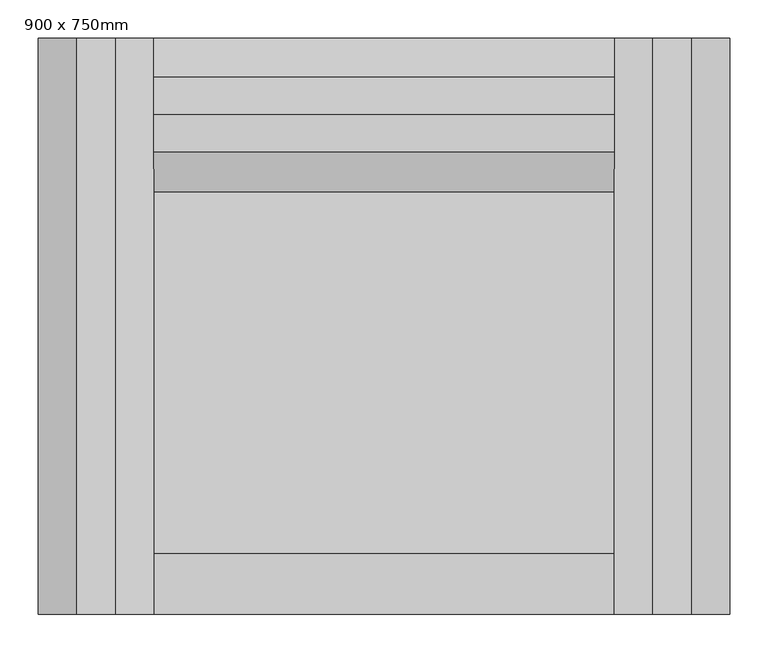
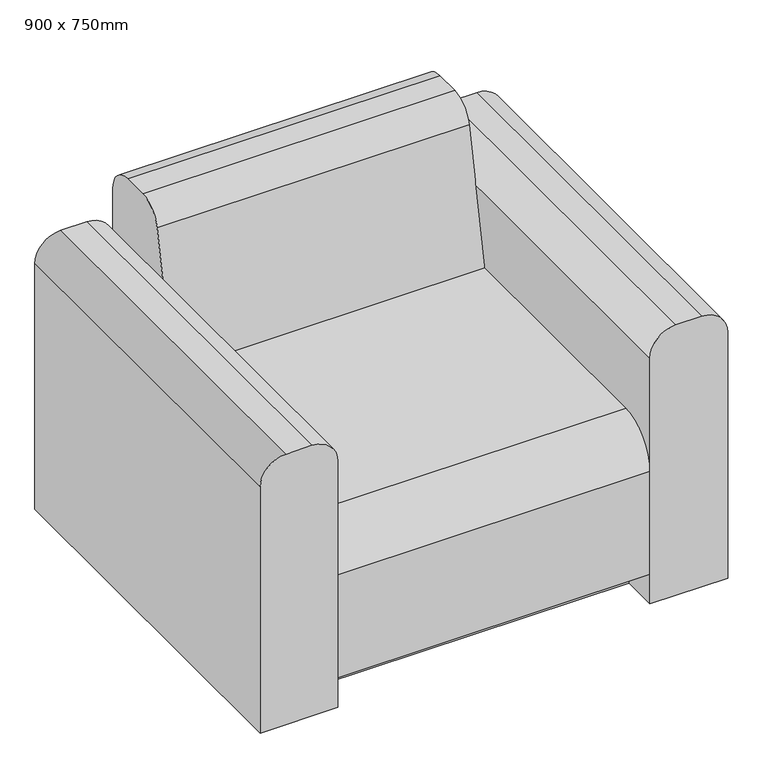
"""IFC4 building model written with IfcOpenShell, lengths in millimetres: furniture geometry, ソファ－I型 : 900 x 750mm."""

import ifcopenshell
import ifcopenshell.guid

model = None  # the IFC model being written
_history = None  # IfcOwnerHistory: only IFC2X3 demands one
_inside = {}  # id of a spatial element -> (the spatial element, [elements in it])
_under = {}  # id of a project, library or spatial element -> (it, [spatial elements below it])
_declared = {}  # id of a project -> (the project, [libraries it declares])
_typed = {}  # id of a type object -> (the type object, [elements of that type])
_made_of = {}  # id of a material, layer set ... -> (it, [elements and type objects made of it])


def new_model(schema):
    """Start an empty IFC model of exactly this schema.

    Asked for "IFC4X3", IfcOpenShell would pick the latest addendum, in which some entities
    have other attributes; the version numbers below select the first issue.
    IFC2X3 requires an IfcOwnerHistory on every rooted entity: one is made here for all.
    """
    global model, _history
    if schema == "IFC4X3":
        model = ifcopenshell.file(schema_version=(4, 3, 0, 0))
    else:
        model = ifcopenshell.file(schema=schema)
    _inside.clear()
    _under.clear()
    _declared.clear()
    _typed.clear()
    _made_of.clear()
    _history = None
    if model.schema == "IFC2X3":
        org = make("IfcOrganization", Name="unknown")
        user = make(
            "IfcPersonAndOrganization",
            ThePerson=make("IfcPerson", FamilyName="unknown"),
            TheOrganization=org,
        )
        app = make(
            "IfcApplication",
            ApplicationDeveloper=org,
            Version="unknown",
            ApplicationFullName="unknown",
            ApplicationIdentifier="unknown",
        )
        _history = make(
            "IfcOwnerHistory",
            OwningUser=user,
            OwningApplication=app,
            ChangeAction="ADDED",
            CreationDate=0,
        )
    return model


def make(cls, **values):
    """One entity of the class cls with the attributes given. An attribute that is None is left unset."""
    return model.create_entity(
        cls, **{name: value for name, value in values.items() if value is not None}
    )


def rooted(cls, **values):
    """An entity with a GlobalId (a new one), such as an element, a storey or a relation."""
    return make(cls, GlobalId=ifcopenshell.guid.new(), OwnerHistory=_history, **values)


def si_unit(unit_type, name, prefix=None):
    """IfcSIUnit, for example si_unit("LENGTHUNIT", "METRE", prefix="MILLI")."""
    return make("IfcSIUnit", UnitType=unit_type, Prefix=prefix, Name=name)


def assignment(units):
    """IfcUnitAssignment: the units of a project."""
    return None if units is None else make("IfcUnitAssignment", Units=units)


def point(xyz):
    """IfcCartesianPoint."""
    return None if xyz is None else make("IfcCartesianPoint", Coordinates=xyz)


def direction(xyz):
    """IfcDirection."""
    return None if xyz is None else make("IfcDirection", DirectionRatios=xyz)


def frame(location, z_axis=None, x_axis=None):
    """IfcAxis2Placement3D, a coordinate frame: its origin and axes. An axis left out is left unset."""
    return make(
        "IfcAxis2Placement3D",
        Location=point(location),
        Axis=direction(z_axis),
        RefDirection=direction(x_axis),
    )


def frame_2d(location, x_axis=None):
    """IfcAxis2Placement2D, a coordinate frame in the plane: its origin and x axis."""
    return make(
        "IfcAxis2Placement2D", Location=point(location), RefDirection=direction(x_axis)
    )


def origin():
    """The frame at (0, 0, 0) with its axes left unset."""
    return frame((0.0, 0.0, 0.0))


def place(relative_to, where):
    """IfcLocalPlacement: puts the frame where relative to a parent placement (None: the world)."""
    return make(
        "IfcLocalPlacement", PlacementRelTo=relative_to, RelativePlacement=where
    )


def context(
    kind, dimensions, precision=None, world=None, true_north=None, identifier=None
):
    """IfcGeometricRepresentationContext, for example the 3D "Model" context."""
    return make(
        "IfcGeometricRepresentationContext",
        ContextIdentifier=identifier,
        ContextType=kind,
        CoordinateSpaceDimension=dimensions,
        Precision=precision,
        WorldCoordinateSystem=world,
        TrueNorth=true_north,
    )


def project(units=None, contexts=None):
    """IfcProject with its units and contexts."""
    return rooted(
        "IfcProject",
        Name="project",
        RepresentationContexts=contexts,
        UnitsInContext=assignment(units),
    )


def spatial(cls, under=None, at=None, **own):
    """A site, building, storey or space (cls), placed at a placement, below another one or the project."""
    s = rooted(cls, ObjectPlacement=at, **own)
    if under is not None:
        _under.setdefault(under.id(), (under, []))[1].append(s)
    return s


def polyline(points):
    """IfcPolyline through the points."""
    return make("IfcPolyline", Points=[point(p) for p in points])


def circle_curve(where, radius):
    """IfcCircle in the frame where."""
    return make("IfcCircle", Position=where, Radius=radius)


def trimmed(basis, trim1, trim2, sense, master):
    """IfcTrimmedCurve: the piece of a basis curve between two trims."""
    return make(
        "IfcTrimmedCurve",
        BasisCurve=basis,
        Trim1=trim1,
        Trim2=trim2,
        SenseAgreement=sense,
        MasterRepresentation=master,
    )


def segment(curve, same_sense, transition):
    """IfcCompositeCurveSegment."""
    return make(
        "IfcCompositeCurveSegment",
        Transition=transition,
        SameSense=same_sense,
        ParentCurve=curve,
    )


def composite_curve(segments, self_intersect=None):
    """IfcCompositeCurve: segments joined end to end."""
    return make("IfcCompositeCurve", Segments=segments, SelfIntersect=self_intersect)


def outline(outer, holes=None, kind="AREA"):
    """IfcArbitraryClosedProfileDef: a profile drawn as a closed curve; with holes, ...WithVoids."""
    if holes is None:
        return make("IfcArbitraryClosedProfileDef", ProfileType=kind, OuterCurve=outer)
    return make(
        "IfcArbitraryProfileDefWithVoids",
        ProfileType=kind,
        OuterCurve=outer,
        InnerCurves=holes,
    )


def extrude(swept, where, along, depth):
    """IfcExtrudedAreaSolid: the profile swept, set in the frame where, extruded along a direction by depth."""
    return make(
        "IfcExtrudedAreaSolid",
        SweptArea=swept,
        Position=where,
        ExtrudedDirection=direction(along),
        Depth=depth,
    )


def shape(context_of_items, identifier, shape_type, items):
    """IfcShapeRepresentation: the items that make up one representation, for example the "Body"."""
    return make(
        "IfcShapeRepresentation",
        ContextOfItems=context_of_items,
        RepresentationIdentifier=identifier,
        RepresentationType=shape_type,
        Items=items,
    )


def source(mapping_origin, context_of_items, identifier, shape_type, items):
    """IfcRepresentationMap: a shape defined once, which mapped items show again and again."""
    return make(
        "IfcRepresentationMap",
        MappingOrigin=mapping_origin,
        MappedRepresentation=shape(context_of_items, identifier, shape_type, items),
    )


def transform(
    local_origin,
    x_axis=None,
    y_axis=None,
    z_axis=None,
    scale=None,
    scale2=None,
    scale3=None,
    uniform=True,
):
    """IfcCartesianTransformationOperator3D, or its non-uniform kind. x_axis, y_axis, z_axis: its Axis1, 2, 3."""
    if uniform:
        return make(
            "IfcCartesianTransformationOperator3D",
            Axis1=direction(x_axis),
            Axis2=direction(y_axis),
            LocalOrigin=point(local_origin),
            Scale=scale,
            Axis3=direction(z_axis),
        )
    return make(
        "IfcCartesianTransformationOperator3DnonUniform",
        Axis1=direction(x_axis),
        Axis2=direction(y_axis),
        LocalOrigin=point(local_origin),
        Scale=scale,
        Axis3=direction(z_axis),
        Scale2=scale2,
        Scale3=scale3,
    )


def mapped(mapping_source, mapping_target):
    """IfcMappedItem: shows the shape of a source again, moved by a transform."""
    return make(
        "IfcMappedItem", MappingSource=mapping_source, MappingTarget=mapping_target
    )


def made_of(thing, what):
    """Note that an element or type object is made of a material, layer set ...; save() writes the relation."""
    if what is not None:
        _made_of.setdefault(what.id(), (what, []))[1].append(thing)
    return thing


def element(
    cls,
    number,
    at=None,
    inside=None,
    cuts=None,
    type_object=None,
    material=None,
    context=None,
    identifier="Body",
    shape_type=None,
    held_by="IfcProductDefinitionShape",
    body=None,
    shapes=None,
    **own,
):
    """One element of the class cls, such as IfcWall. Its Tag is "e" and its number.

    at: its placement. inside: the storey or other place that contains it. cuts: it is an
    opening in that element (IfcRelVoidsElement). A single representation is given by context,
    identifier, shape_type and body (its items); several are given by shapes. held_by: the class
    of the entity that holds the representations. save() writes the other relations.
    """
    e = rooted(cls, Tag="e%d" % number, ObjectPlacement=at, **own)
    if body is not None:
        shapes = [shape(context, identifier, shape_type, body)]
    if shapes is not None:
        e.Representation = make(held_by, Representations=shapes)
    if inside is not None:
        _inside.setdefault(inside.id(), (inside, []))[1].append(e)
    if cuts is not None:
        rooted(
            "IfcRelVoidsElement", RelatingBuildingElement=cuts, RelatedOpeningElement=e
        )
    if type_object is not None:
        _typed.setdefault(type_object.id(), (type_object, []))[1].append(e)
    return made_of(e, material)


def aggregate(whole, parts):
    """IfcRelAggregates: a whole, such as a stair, and the parts it consists of."""
    return rooted("IfcRelAggregates", RelatingObject=whole, RelatedObjects=parts)


def save(model, path):
    """Write the relations noted so far, then the file.

    IfcRelAggregates (storeys below a building ...), IfcRelContainedInSpatialStructure (elements
    in a storey), IfcRelDefinesByType, IfcRelAssociatesMaterial and IfcRelDeclares: one each for
    every whole, place, type object, material and project.
    """
    for whole, parts in _under.values():
        aggregate(whole, parts)
    for where, things in _inside.values():
        rooted(
            "IfcRelContainedInSpatialStructure",
            RelatedElements=things,
            RelatingStructure=where,
        )
    for kind, things in _typed.values():
        rooted("IfcRelDefinesByType", RelatedObjects=things, RelatingType=kind)
    for what, things in _made_of.values():
        rooted("IfcRelAssociatesMaterial", RelatedObjects=things, RelatingMaterial=what)
    for by, libraries in _declared.values():
        rooted("IfcRelDeclares", RelatingContext=by, RelatedDefinitions=libraries)
    model.write(path)


def furniture_900_x_750mm_ff71e519(model_context):
    return source(origin(), model_context, "Body", "SweptSolid", [
        extrude(outline(composite_curve([segment(trimmed(circle_curve(frame_2d((500.0, -400.0)), 50.0), [point((550.0, -400.0))], [point((500.0, -450.0))], False, "CARTESIAN"), True, "CONTINUOUS"), segment(polyline([(500.0, -450.0), (0.0, -450.0), (0.0, -300.0), (500.0, -300.0)]), True, "CONTINUOUS"), segment(trimmed(circle_curve(frame_2d((500.0, -350.0)), 50.0), [point((500.0, -300.0))], [point((550.0, -350.0))], False, "CARTESIAN"), True, "CONTINUOUS"), segment(polyline([(550.0, -350.0), (550.0, -400.0)]), True, "CONTINUOUS")], self_intersect=False)), frame((0.0, -375.0, 0.0), z_axis=(0.0, 1.0, 0.0), x_axis=(0.0, 0.0, 1.0)), (0.0, 0.0, 1.0), 750.0),
        extrude(outline(composite_curve([segment(polyline([(550.0, 400.0), (550.0, 350.0)]), True, "CONTINUOUS"), segment(trimmed(circle_curve(frame_2d((500.0, 350.0)), 50.0), [point((550.0, 350.0))], [point((500.0, 300.0))], False, "CARTESIAN"), True, "CONTINUOUS"), segment(polyline([(500.0, 300.0), (0.0, 300.0), (0.0, 450.0), (500.0, 450.0)]), True, "CONTINUOUS"), segment(trimmed(circle_curve(frame_2d((500.0, 400.0)), 50.0), [point((500.0, 450.0))], [point((550.0, 400.0))], False, "CARTESIAN"), True, "CONTINUOUS")], self_intersect=False)), frame((0.0, -375.0, 0.0), z_axis=(0.0, 1.0, 0.0), x_axis=(0.0, 0.0, 1.0)), (0.0, 0.0, 1.0), 750.0),
        extrude(outline(composite_curve([segment(trimmed(circle_curve(frame_2d((275.9901951, 600.0)), 50.0), [point((226.9611614, 609.8058068))], [point((275.9901951, 650.0))], False, "CARTESIAN"), True, "CONTINUOUS"), segment(polyline([(275.9901951, 650.0), (325.0, 650.0)]), True, "CONTINUOUS"), segment(trimmed(circle_curve(frame_2d((325.0, 600.0)), 50.0), [point((325.0, 650.0))], [point((375.0, 600.0))], False, "CARTESIAN"), True, "CONTINUOUS"), segment(polyline([(375.0, 600.0), (375.0, 0.0), (-305.0, 0.0), (-305.0, 60.0), (-375.0, 60.0), (-375.0, 270.0)]), True, "CONTINUOUS"), segment(trimmed(circle_curve(frame_2d((-295.0, 270.0)), 80.0), [point((-375.0, 270.0))], [point((-295.0, 350.0))], False, "CARTESIAN"), True, "CONTINUOUS"), segment(polyline([(-295.0, 350.0), (175.0, 350.0), (226.9611614, 609.8058068)]), True, "CONTINUOUS")], self_intersect=False)), frame((-300.0, 0.0, 0.0), z_axis=(1.0, 0.0, 0.0), x_axis=(0.0, 1.0, 0.0)), (0.0, 0.0, 1.0), 600.0),
    ])


if __name__ == "__main__":
    model = new_model("IFC4")
    model_context = context("Model", 3, world=origin())
    ifc_project = project(units=[si_unit("LENGTHUNIT", "METRE", prefix="MILLI")], contexts=[model_context])
    site = spatial("IfcSite", under=ifc_project)
    building = spatial("IfcBuilding", under=site)
    placement = place(None, origin())
    furniture_900_x_750mm_shape = furniture_900_x_750mm_ff71e519(model_context)
    element("IfcFurniture", 1, ObjectType="ソファ－I型 : 900 x 750mm", at=placement, inside=building, context=model_context, shape_type="MappedRepresentation", body=[
        mapped(furniture_900_x_750mm_shape, transform((0.0, 0.0, 0.0), x_axis=(1.0, 0.0, 0.0), y_axis=(0.0, 1.0, 0.0), z_axis=(0.0, 0.0, 1.0))),
    ])
    save(model, "model.ifc")

# Revit data of these elements
# Type "ソファ－I型 : 900 x 750mm"
#   Keynote = "12490.Y1"
#   座面高さ = 350 mm
#   幅 = 900 mm
#   奥行き = 750 mm
#   本体 = モチアミ - 無地 - グレー
#   Default Elevation = 0
# Element 1 (IfcFurniture, "ソファ－I型 : 900 x 750mm")
#   Materials on its faces: "モチアミ - 無地 - グレー"
# Materials
#   "モチアミ - 無地 - グレー": class "モチアミ", colour RGB 65 63 65, transparency 0, Cost = 0
